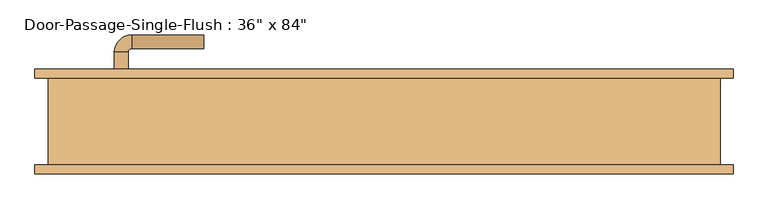
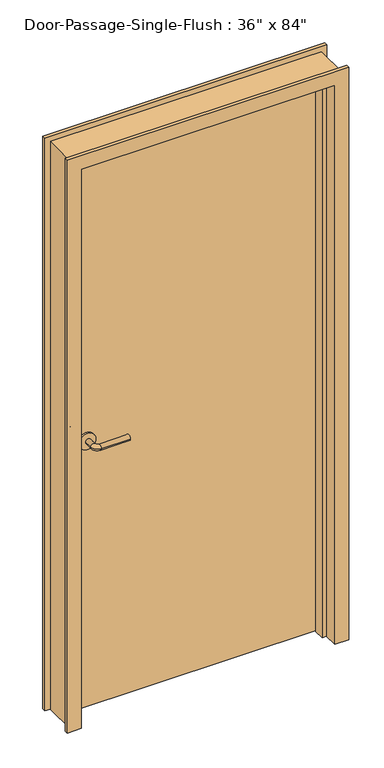
"""IFC4 building model written with IfcOpenShell, lengths in millimetres: door geometry."""

from ifc_helpers import new_model, si_unit, point, frame, frame_2d, origin, origin_with_axes, place, context, project, spatial, polyline, circle_curve, ellipse_curve, trimmed, segment, composite_curve, outline, extrude, faceted_brep, source, transform, mapped, element, save
from ifc_brep_helpers import plane_surface, cylinder_surface, revolved_surface, advanced_brep


def door_12b10c6a(model_context):
    return source(origin(), model_context, "Body", "SolidModel", [
        advanced_brep(
        [(-392.190625, 17.4, 1016.0), (-372.190625, 17.4, 1016.0), (-372.190625, -12.6, 1016.0), (-392.190625, -12.6, 1016.0), (-367.190625, -17.6, 1016.0), (-367.190625, -37.6, 1016.0), (-262.190625, -37.6, 1016.0), (-262.190625, -17.6, 1016.0)],
        [
            (0, 1, circle_curve(frame((-382.190625, 17.4, 1016.0), z_axis=(0.0, 1.0, 0.0), x_axis=(1.0, 0.0, 0.0)), 10.0)),
            (1, 0, circle_curve(frame((-382.190625, 17.4, 1016.0), z_axis=(0.0, 1.0, 0.0), x_axis=(1.0, 0.0, 0.0)), 10.0)),
            (1, 2),
            (2, 3, circle_curve(frame((-382.190625, -12.6, 1016.0), z_axis=(0.0, 1.0, 0.0), x_axis=(1.0, 0.0, 0.0)), 10.0)),
            (3, 0),
            (3, 2, circle_curve(frame((-382.190625, -12.6, 1016.0), z_axis=(0.0, 1.0, 0.0), x_axis=(1.0, 0.0, 0.0)), 10.0)),
            (4, 5, circle_curve(frame((-367.190625, -27.6, 1016.0), z_axis=(-1.0, 0.0, 0.0), x_axis=(0.0, 1.0, 0.0)), 10.0)),
            (5, 3, circle_curve(frame((-367.190625, -12.6, 1016.0), z_axis=(0.0, 0.0, -1.0), x_axis=(-1.0, 0.0, 0.0)), 25.0)),
            (2, 4, circle_curve(frame((-367.190625, -12.6, 1016.0), z_axis=(0.0, 0.0, 1.0), x_axis=(-1.0, 0.0, 0.0)), 5.0)),
            (5, 4, circle_curve(frame((-367.190625, -27.6, 1016.0), z_axis=(-1.0, 0.0, 0.0), x_axis=(0.0, 1.0, 0.0)), 10.0)),
            (6, 7, circle_curve(frame((-262.190625, -27.6, 1016.0), z_axis=(1.0, 0.0, 0.0), x_axis=(0.0, 1.0, 0.0)), 10.0)),
            (7, 6, circle_curve(frame((-262.190625, -27.6, 1016.0), z_axis=(1.0, 0.0, 0.0), x_axis=(0.0, 1.0, 0.0)), 10.0)),
            (4, 7),
            (6, 5),
        ],
        [
            plane_surface(frame((-382.190625, 17.4, 1016.0), z_axis=(0.0, 1.0, 0.0), x_axis=(0.0, 0.0, 1.0))),
            cylinder_surface(frame((-382.190625, 17.4, 1016.0), z_axis=(0.0, 1.0, 0.0), x_axis=(1.0, 0.0, 0.0)), 10.0),
            revolved_surface(trimmed(ellipse_curve(frame((-382.190625, -12.6, 1016.0), z_axis=(0.0, -1.0, 0.0), x_axis=(1.0, 0.0, 0.0)), 10.0, 10.0), [point((-392.190625, -12.6, 1016.0))], [point((-372.190625, -12.6, 1016.0))], True, "CARTESIAN"), (-367.190625, -12.6, 1016.0), (0.0, 0.0, -1.0)),
            revolved_surface(trimmed(ellipse_curve(frame((-382.190625, -12.6, 1016.0), z_axis=(0.0, -1.0, 0.0), x_axis=(1.0, 0.0, 0.0)), 10.0, 10.0), [point((-372.190625, -12.6, 1016.0))], [point((-392.190625, -12.6, 1016.0))], True, "CARTESIAN"), (-367.190625, -12.6, 1016.0), (0.0, 0.0, -1.0)),
            plane_surface(frame((-262.190625, -27.6, 1016.0), z_axis=(1.0, 0.0, 0.0), x_axis=(0.0, 0.0, 1.0))),
            cylinder_surface(frame((-367.190625, -27.6, 1016.0), z_axis=(-1.0, 0.0, 0.0), x_axis=(0.0, 1.0, 0.0)), 10.0),
        ],
        [
            (0, [[1, 2]]),
            (1, [[3, 4, 5, -2]]),
            (1, [[-5, 6, -3, -1]]),
            (2, [[7, 8, -4, 9]]),
            (3, [[10, -9, -6, -8]]),
            (4, [[11, 12]]),
            (5, [[13, -11, 14, -7]]),
            (5, [[-14, -12, -13, -10]]),
        ],
    ),
        extrude(outline(composite_curve([segment(trimmed(circle_curve(frame_2d((1016.0, -384.690625)), 30.0), [point((1016.0, -414.690625))], [point((1016.0, -354.690625))], False, "CARTESIAN"), True, "CONTINUOUS"), segment(trimmed(circle_curve(frame_2d((1016.0, -384.690625)), 30.0), [point((1016.0, -354.690625))], [point((1016.0, -414.690625))], False, "CARTESIAN"), True, "CONTINUOUS")], self_intersect=False)), frame((0.0, 17.4, 0.0), z_axis=(0.0, 1.0, 0.0), x_axis=(0.0, 0.0, 1.0)), (0.0, 0.0, 1.0), 8.0),
        advanced_brep(
        [(-392.190625, 77.85, 1016.0), (-372.190625, 77.85, 1016.0), (-392.190625, 107.85, 1016.0), (-372.190625, 107.85, 1016.0), (-367.190625, 112.85, 1016.0), (-367.190625, 132.85, 1016.0), (-262.190625, 132.85, 1016.0), (-262.190625, 112.85, 1016.0)],
        [
            (0, 1, circle_curve(frame((-382.190625, 77.85, 1016.0), z_axis=(0.0, -1.0, 0.0), x_axis=(1.0, 0.0, 0.0)), 10.0)),
            (1, 0, circle_curve(frame((-382.190625, 77.85, 1016.0), z_axis=(0.0, -1.0, 0.0), x_axis=(1.0, 0.0, 0.0)), 10.0)),
            (0, 2),
            (2, 3, circle_curve(frame((-382.190625, 107.85, 1016.0), z_axis=(0.0, -1.0, 0.0), x_axis=(1.0, 0.0, 0.0)), 10.0)),
            (3, 1),
            (3, 2, circle_curve(frame((-382.190625, 107.85, 1016.0), z_axis=(0.0, -1.0, 0.0), x_axis=(1.0, 0.0, 0.0)), 10.0)),
            (4, 3, circle_curve(frame((-367.190625, 107.85, 1016.0), z_axis=(0.0, 0.0, 1.0), x_axis=(-1.0, 0.0, 0.0)), 5.0)),
            (2, 5, circle_curve(frame((-367.190625, 107.85, 1016.0), z_axis=(0.0, 0.0, -1.0), x_axis=(-1.0, 0.0, 0.0)), 25.0)),
            (5, 4, circle_curve(frame((-367.190625, 122.85, 1016.0), z_axis=(-1.0, 0.0, 0.0), x_axis=(0.0, -1.0, 0.0)), 10.0)),
            (4, 5, circle_curve(frame((-367.190625, 122.85, 1016.0), z_axis=(-1.0, 0.0, 0.0), x_axis=(0.0, -1.0, 0.0)), 10.0)),
            (6, 7, circle_curve(frame((-262.190625, 122.85, 1016.0), z_axis=(1.0, 0.0, 0.0), x_axis=(0.0, -1.0, 0.0)), 10.0)),
            (7, 6, circle_curve(frame((-262.190625, 122.85, 1016.0), z_axis=(1.0, 0.0, 0.0), x_axis=(0.0, -1.0, 0.0)), 10.0)),
            (5, 6),
            (7, 4),
        ],
        [
            plane_surface(frame((-382.190625, 77.85, 1016.0), z_axis=(0.0, -1.0, 0.0), x_axis=(0.0, 0.0, 1.0))),
            cylinder_surface(frame((-382.190625, 77.85, 1016.0), z_axis=(0.0, -1.0, 0.0), x_axis=(1.0, 0.0, 0.0)), 10.0),
            revolved_surface(trimmed(ellipse_curve(frame((-382.190625, 107.85, 1016.0), z_axis=(0.0, -1.0, 0.0), x_axis=(1.0, 0.0, 0.0)), 10.0, 10.0), [point((-392.190625, 107.85, 1016.0))], [point((-372.190625, 107.85, 1016.0))], True, "CARTESIAN"), (-367.190625, 107.85, 1016.0), (0.0, 0.0, -1.0)),
            revolved_surface(trimmed(ellipse_curve(frame((-382.190625, 107.85, 1016.0), z_axis=(0.0, -1.0, 0.0), x_axis=(1.0, 0.0, 0.0)), 10.0, 10.0), [point((-372.190625, 107.85, 1016.0))], [point((-392.190625, 107.85, 1016.0))], True, "CARTESIAN"), (-367.190625, 107.85, 1016.0), (0.0, 0.0, -1.0)),
            plane_surface(frame((-262.190625, 122.85, 1016.0), z_axis=(1.0, 0.0, 0.0), x_axis=(0.0, 0.0, 1.0))),
            cylinder_surface(frame((-367.190625, 122.85, 1016.0), z_axis=(-1.0, 0.0, 0.0), x_axis=(0.0, -1.0, 0.0)), 10.0),
        ],
        [
            (0, [[1, 2]]),
            (1, [[-1, 3, 4, 5]]),
            (1, [[-2, -5, 6, -3]]),
            (2, [[7, -4, 8, 9]]),
            (3, [[-8, -6, -7, 10]]),
            (4, [[11, 12]]),
            (5, [[-9, 13, -12, 14]]),
            (5, [[-10, -14, -11, -13]]),
        ],
    ),
        extrude(outline(composite_curve([segment(trimmed(circle_curve(frame_2d((1016.0, -384.690625)), 30.0), [point((1016.0, -414.690625))], [point((1016.0, -354.690625))], False, "CARTESIAN"), True, "CONTINUOUS"), segment(trimmed(circle_curve(frame_2d((1016.0, -384.690625)), 30.0), [point((1016.0, -354.690625))], [point((1016.0, -414.690625))], False, "CARTESIAN"), True, "CONTINUOUS")], self_intersect=False)), frame((0.0, 69.85, 0.0), z_axis=(0.0, 1.0, 0.0), x_axis=(0.0, 0.0, 1.0)), (0.0, 0.0, 1.0), 8.0),
        faceted_brep([(457.2, 82.55, 0.0), (508.0, 82.55, 0.0), (508.0, 69.85, 0.0), (488.95, 69.85, 0.0), (488.95, -57.15, 0.0), (508.0, -57.15, 0.0), (508.0, -69.85, 0.0), (457.2, -69.85, 0.0), (457.2, -17.4625, 0.0), (441.325, -17.4625, 0.0), (441.325, 20.6375, 0.0), (457.2, 20.6375, 0.0), (457.2, 82.55, 2133.6), (-457.2, 82.55, 2133.6), (-457.2, 82.55, 0.0), (-508.0, 82.55, 0.0), (-508.0, 82.55, 2184.4), (508.0, 82.55, 2184.4), (508.0, 69.85, 2184.4), (-508.0, 69.85, 2184.4), (-508.0, 69.85, 0.0), (-488.95, 69.85, 0.0), (-488.95, 69.85, 2165.35), (488.95, 69.85, 2165.35), (488.95, -57.15, 2165.35), (-488.95, -57.15, 2165.35), (-488.95, -57.15, 0.0), (-508.0, -57.15, 0.0), (-508.0, -57.15, 2184.4), (508.0, -57.15, 2184.4), (508.0, -69.85, 2184.4), (-508.0, -69.85, 2184.4), (-508.0, -69.85, 0.0), (-457.2, -69.85, 0.0), (-457.2, -69.85, 2133.6), (457.2, -69.85, 2133.6), (457.2, -17.4625, 2133.6), (-457.2, -17.4625, 2133.6), (-457.2, -17.4625, 0.0), (-441.325, -17.4625, 0.0), (-441.325, -17.4625, 2117.725), (441.325, -17.4625, 2117.725), (441.325, 20.6375, 2117.725), (-441.325, 20.6375, 2117.725), (-441.325, 20.6375, 0.0), (-457.2, 20.6375, 0.0), (-457.2, 20.6375, 2133.6), (457.2, 20.6375, 2133.6)], [[[0, 1, 2, 3, 4, 5, 6, 7, 8, 9, 10, 11]], [[1, 0, 12, 13, 14, 15, 16, 17]], [[2, 1, 17, 18]], [[3, 2, 18, 19, 20, 21, 22, 23]], [[4, 3, 23, 24]], [[5, 4, 24, 25, 26, 27, 28, 29]], [[6, 5, 29, 30]], [[7, 6, 30, 31, 32, 33, 34, 35]], [[8, 7, 35, 36]], [[9, 8, 36, 37, 38, 39, 40, 41]], [[10, 9, 41, 42]], [[11, 10, 42, 43, 44, 45, 46, 47]], [[0, 11, 47, 12]], [[18, 17, 16, 19]], [[24, 23, 22, 25]], [[30, 29, 28, 31]], [[36, 35, 34, 37]], [[42, 41, 40, 43]], [[12, 47, 46, 13]], [[14, 45, 44, 39, 38, 33, 32, 27, 26, 21, 20, 15]], [[19, 16, 15, 20]], [[25, 22, 21, 26]], [[31, 28, 27, 32]], [[37, 34, 33, 38]], [[43, 40, 39, 44]], [[13, 46, 45, 14]]]),
        extrude(outline(polyline([(457.2, 25.4), (-457.2, 25.4), (-457.2, 69.85), (457.2, 69.85), (457.2, 25.4)])), origin_with_axes(), (0.0, 0.0, 1.0), 2133.6),
    ])


if __name__ == "__main__":
    model = new_model("IFC4")
    model_context = context("Model", 3, world=origin())
    ifc_project = project(units=[si_unit("LENGTHUNIT", "METRE", prefix="MILLI")], contexts=[model_context])
    site = spatial("IfcSite", under=ifc_project)
    building = spatial("IfcBuilding", under=site)
    placement = place(None, origin())
    door_shape = door_12b10c6a(model_context)
    element("IfcDoor", 1, ObjectType="Door-Passage-Single-Flush : 36\" x 84\"", at=placement, inside=building, context=model_context, shape_type="MappedRepresentation", body=[
        mapped(door_shape, transform((0.0, 0.0, 0.0), x_axis=(1.0, 0.0, 0.0), y_axis=(0.0, 1.0, 0.0), z_axis=(0.0, 0.0, 1.0))),
    ])
    save(model, "model.ifc")

# Revit data of these elements
# Type "Door-Passage-Single-Flush : 36\" x 84\""
#   Type Mark = "1"
#   Assembly Code = "B2030200"
#   Analytic Construction = "Wooden"
#   Thickness = 0' - 1 3/4"
#   Thermal Resistance (R) = 2.5876 (h·ft²·°F)/BTU
#   Swing Angle [instance default] = 90.00°
#   Strike Height = 3' - 4"
#   Rough Width [instance default] = 3' - 4"
#   Rough Height [instance default] = 7' - 4"
#   MF Opening Height [instance default] = 0' - 4"
#   MF Opening Width [instance default] = 0' - 4"
#   Inset Calculate [instance default] = 0' - 4"
#   Masonry Inset [instance default] = 0' - 1"
#   Height = 7' - 0"
#   Width = 3' - 0"
#   Heat Transfer Coefficient (U) = 0.3865 BTU/(h·ft²·°F)
#   Masonry Frame Depth = 0' - 5 3/4"
#   Function = 0
#   Masonry Frame [instance default] = yes
#   Function = 1
#   Dry Wall Frame [instance default] = no
#   Panel Material = Wood - Birch
#   Frame Material = Metal - Paint Finish - Grey
#   Door Handle Material = Aluminum
#   Visual Light Transmittance = 0
#   Solar Heat Gain Coefficient = 0
#   Wall Closure = (empty or 0)
# Element 1 (IfcDoor, "Door-Passage-Single-Flush : 36\" x 84\"")
#   Rough Width = 3' - 2 1/2"
#   Rough Height = 7' - 1 1/4"
#   MF Opening Height = 0' - 1 1/4"
#   MF Opening Width = 0' - 2 1/2"
#   Inset Calculate = 0' - 3"
#   Masonry Frame = no
#   Dry Wall Frame = yes
#   Materials on its faces: "Metal - Paint Finish - Grey", "Aluminum", "Wood - Birch"
# Materials
#   "Wood - Birch": class "Unassigned", colour RGB 224 178 126, transparency 0
#   "Metal - Paint Finish - Grey": class "Paint", colour RGB 104 104 104, transparency 0, Cost = 0
#   "Aluminum": class "Metal", colour RGB 120 120 120, transparency 0, Description = "Aluminum 6061", Cost = 0
